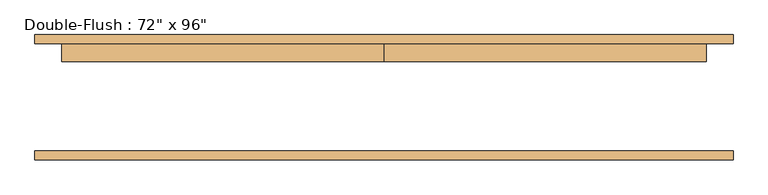
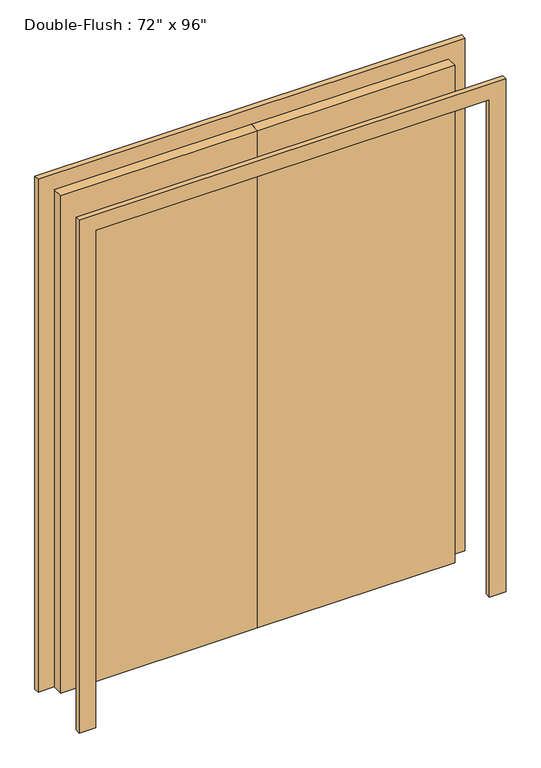
"""IFC4 building model written with IfcOpenShell, lengths in millimetres: door geometry."""

import ifcopenshell
import ifcopenshell.guid

model = None  # the IFC model being written
_history = None  # IfcOwnerHistory: only IFC2X3 demands one
_inside = {}  # id of a spatial element -> (the spatial element, [elements in it])
_under = {}  # id of a project, library or spatial element -> (it, [spatial elements below it])
_declared = {}  # id of a project -> (the project, [libraries it declares])
_typed = {}  # id of a type object -> (the type object, [elements of that type])
_made_of = {}  # id of a material, layer set ... -> (it, [elements and type objects made of it])


def new_model(schema):
    """Start an empty IFC model of exactly this schema.

    Asked for "IFC4X3", IfcOpenShell would pick the latest addendum, in which some entities
    have other attributes; the version numbers below select the first issue.
    IFC2X3 requires an IfcOwnerHistory on every rooted entity: one is made here for all.
    """
    global model, _history
    if schema == "IFC4X3":
        model = ifcopenshell.file(schema_version=(4, 3, 0, 0))
    else:
        model = ifcopenshell.file(schema=schema)
    _inside.clear()
    _under.clear()
    _declared.clear()
    _typed.clear()
    _made_of.clear()
    _history = None
    if model.schema == "IFC2X3":
        org = make("IfcOrganization", Name="unknown")
        user = make(
            "IfcPersonAndOrganization",
            ThePerson=make("IfcPerson", FamilyName="unknown"),
            TheOrganization=org,
        )
        app = make(
            "IfcApplication",
            ApplicationDeveloper=org,
            Version="unknown",
            ApplicationFullName="unknown",
            ApplicationIdentifier="unknown",
        )
        _history = make(
            "IfcOwnerHistory",
            OwningUser=user,
            OwningApplication=app,
            ChangeAction="ADDED",
            CreationDate=0,
        )
    return model


def make(cls, **values):
    """One entity of the class cls with the attributes given. An attribute that is None is left unset."""
    return model.create_entity(
        cls, **{name: value for name, value in values.items() if value is not None}
    )


def rooted(cls, **values):
    """An entity with a GlobalId (a new one), such as an element, a storey or a relation."""
    return make(cls, GlobalId=ifcopenshell.guid.new(), OwnerHistory=_history, **values)


def si_unit(unit_type, name, prefix=None):
    """IfcSIUnit, for example si_unit("LENGTHUNIT", "METRE", prefix="MILLI")."""
    return make("IfcSIUnit", UnitType=unit_type, Prefix=prefix, Name=name)


def assignment(units):
    """IfcUnitAssignment: the units of a project."""
    return None if units is None else make("IfcUnitAssignment", Units=units)


def point(xyz):
    """IfcCartesianPoint."""
    return None if xyz is None else make("IfcCartesianPoint", Coordinates=xyz)


def direction(xyz):
    """IfcDirection."""
    return None if xyz is None else make("IfcDirection", DirectionRatios=xyz)


def frame(location, z_axis=None, x_axis=None):
    """IfcAxis2Placement3D, a coordinate frame: its origin and axes. An axis left out is left unset."""
    return make(
        "IfcAxis2Placement3D",
        Location=point(location),
        Axis=direction(z_axis),
        RefDirection=direction(x_axis),
    )


def origin():
    """The frame at (0, 0, 0) with its axes left unset."""
    return frame((0.0, 0.0, 0.0))


def origin_with_axes():
    """The frame at (0, 0, 0) with the z axis (0, 0, 1) and the x axis (1, 0, 0) written out."""
    return frame((0.0, 0.0, 0.0), z_axis=(0.0, 0.0, 1.0), x_axis=(1.0, 0.0, 0.0))


def place(relative_to, where):
    """IfcLocalPlacement: puts the frame where relative to a parent placement (None: the world)."""
    return make(
        "IfcLocalPlacement", PlacementRelTo=relative_to, RelativePlacement=where
    )


def context(
    kind, dimensions, precision=None, world=None, true_north=None, identifier=None
):
    """IfcGeometricRepresentationContext, for example the 3D "Model" context."""
    return make(
        "IfcGeometricRepresentationContext",
        ContextIdentifier=identifier,
        ContextType=kind,
        CoordinateSpaceDimension=dimensions,
        Precision=precision,
        WorldCoordinateSystem=world,
        TrueNorth=true_north,
    )


def project(units=None, contexts=None):
    """IfcProject with its units and contexts."""
    return rooted(
        "IfcProject",
        Name="project",
        RepresentationContexts=contexts,
        UnitsInContext=assignment(units),
    )


def spatial(cls, under=None, at=None, **own):
    """A site, building, storey or space (cls), placed at a placement, below another one or the project."""
    s = rooted(cls, ObjectPlacement=at, **own)
    if under is not None:
        _under.setdefault(under.id(), (under, []))[1].append(s)
    return s


def polyline(points):
    """IfcPolyline through the points."""
    return make("IfcPolyline", Points=[point(p) for p in points])


def outline(outer, holes=None, kind="AREA"):
    """IfcArbitraryClosedProfileDef: a profile drawn as a closed curve; with holes, ...WithVoids."""
    if holes is None:
        return make("IfcArbitraryClosedProfileDef", ProfileType=kind, OuterCurve=outer)
    return make(
        "IfcArbitraryProfileDefWithVoids",
        ProfileType=kind,
        OuterCurve=outer,
        InnerCurves=holes,
    )


def extrude(swept, where, along, depth):
    """IfcExtrudedAreaSolid: the profile swept, set in the frame where, extruded along a direction by depth."""
    return make(
        "IfcExtrudedAreaSolid",
        SweptArea=swept,
        Position=where,
        ExtrudedDirection=direction(along),
        Depth=depth,
    )


def shape(context_of_items, identifier, shape_type, items):
    """IfcShapeRepresentation: the items that make up one representation, for example the "Body"."""
    return make(
        "IfcShapeRepresentation",
        ContextOfItems=context_of_items,
        RepresentationIdentifier=identifier,
        RepresentationType=shape_type,
        Items=items,
    )


def source(mapping_origin, context_of_items, identifier, shape_type, items):
    """IfcRepresentationMap: a shape defined once, which mapped items show again and again."""
    return make(
        "IfcRepresentationMap",
        MappingOrigin=mapping_origin,
        MappedRepresentation=shape(context_of_items, identifier, shape_type, items),
    )


def transform(
    local_origin,
    x_axis=None,
    y_axis=None,
    z_axis=None,
    scale=None,
    scale2=None,
    scale3=None,
    uniform=True,
):
    """IfcCartesianTransformationOperator3D, or its non-uniform kind. x_axis, y_axis, z_axis: its Axis1, 2, 3."""
    if uniform:
        return make(
            "IfcCartesianTransformationOperator3D",
            Axis1=direction(x_axis),
            Axis2=direction(y_axis),
            LocalOrigin=point(local_origin),
            Scale=scale,
            Axis3=direction(z_axis),
        )
    return make(
        "IfcCartesianTransformationOperator3DnonUniform",
        Axis1=direction(x_axis),
        Axis2=direction(y_axis),
        LocalOrigin=point(local_origin),
        Scale=scale,
        Axis3=direction(z_axis),
        Scale2=scale2,
        Scale3=scale3,
    )


def mapped(mapping_source, mapping_target):
    """IfcMappedItem: shows the shape of a source again, moved by a transform."""
    return make(
        "IfcMappedItem", MappingSource=mapping_source, MappingTarget=mapping_target
    )


def made_of(thing, what):
    """Note that an element or type object is made of a material, layer set ...; save() writes the relation."""
    if what is not None:
        _made_of.setdefault(what.id(), (what, []))[1].append(thing)
    return thing


def element(
    cls,
    number,
    at=None,
    inside=None,
    cuts=None,
    type_object=None,
    material=None,
    context=None,
    identifier="Body",
    shape_type=None,
    held_by="IfcProductDefinitionShape",
    body=None,
    shapes=None,
    **own,
):
    """One element of the class cls, such as IfcWall. Its Tag is "e" and its number.

    at: its placement. inside: the storey or other place that contains it. cuts: it is an
    opening in that element (IfcRelVoidsElement). A single representation is given by context,
    identifier, shape_type and body (its items); several are given by shapes. held_by: the class
    of the entity that holds the representations. save() writes the other relations.
    """
    e = rooted(cls, Tag="e%d" % number, ObjectPlacement=at, **own)
    if body is not None:
        shapes = [shape(context, identifier, shape_type, body)]
    if shapes is not None:
        e.Representation = make(held_by, Representations=shapes)
    if inside is not None:
        _inside.setdefault(inside.id(), (inside, []))[1].append(e)
    if cuts is not None:
        rooted(
            "IfcRelVoidsElement", RelatingBuildingElement=cuts, RelatedOpeningElement=e
        )
    if type_object is not None:
        _typed.setdefault(type_object.id(), (type_object, []))[1].append(e)
    return made_of(e, material)


def aggregate(whole, parts):
    """IfcRelAggregates: a whole, such as a stair, and the parts it consists of."""
    return rooted("IfcRelAggregates", RelatingObject=whole, RelatedObjects=parts)


def save(model, path):
    """Write the relations noted so far, then the file.

    IfcRelAggregates (storeys below a building ...), IfcRelContainedInSpatialStructure (elements
    in a storey), IfcRelDefinesByType, IfcRelAssociatesMaterial and IfcRelDeclares: one each for
    every whole, place, type object, material and project.
    """
    for whole, parts in _under.values():
        aggregate(whole, parts)
    for where, things in _inside.values():
        rooted(
            "IfcRelContainedInSpatialStructure",
            RelatedElements=things,
            RelatingStructure=where,
        )
    for kind, things in _typed.values():
        rooted("IfcRelDefinesByType", RelatedObjects=things, RelatingType=kind)
    for what, things in _made_of.values():
        rooted("IfcRelAssociatesMaterial", RelatedObjects=things, RelatingMaterial=what)
    for by, libraries in _declared.values():
        rooted("IfcRelDeclares", RelatingContext=by, RelatedDefinitions=libraries)
    model.write(path)


def door_6d7ee948(model_context):
    return source(origin(), model_context, "Body", "SweptSolid", [
        extrude(outline(polyline([(0.0, 152.4), (914.4, 152.4), (914.4, 101.6), (0.0, 101.6), (0.0, 152.4)])), origin_with_axes(), (0.0, 0.0, 1.0), 2438.4),
        extrude(outline(polyline([(-914.4, 152.4), (0.0, 152.4), (0.0, 101.6), (-914.4, 101.6), (-914.4, 152.4)])), origin_with_axes(), (0.0, 0.0, 1.0), 2438.4),
        extrude(outline(polyline([(2438.4, -914.4), (2438.4, 914.4), (0.0, 914.4), (0.0, 990.6), (2514.6, 990.6), (2514.6, -990.6), (0.0, -990.6), (0.0, -914.4), (2438.4, -914.4)])), frame((0.0, -177.8, 0.0), z_axis=(0.0, 1.0, 0.0), x_axis=(0.0, 0.0, 1.0)), (0.0, 0.0, 1.0), 25.4),
        extrude(outline(polyline([(2438.4, -914.4), (2438.4, 914.4), (0.0, 914.4), (0.0, 990.6), (2514.6, 990.6), (2514.6, -990.6), (0.0, -990.6), (0.0, -914.4), (2438.4, -914.4)])), frame((0.0, 152.4, 0.0), z_axis=(0.0, 1.0, 0.0), x_axis=(0.0, 0.0, 1.0)), (0.0, 0.0, 1.0), 25.4),
    ])


if __name__ == "__main__":
    model = new_model("IFC4")
    model_context = context("Model", 3, world=origin())
    ifc_project = project(units=[si_unit("LENGTHUNIT", "METRE", prefix="MILLI")], contexts=[model_context])
    site = spatial("IfcSite", under=ifc_project)
    building = spatial("IfcBuilding", under=site)
    placement = place(None, origin())
    door_shape = door_6d7ee948(model_context)
    element("IfcDoor", 1, ObjectType="Double-Flush : 72\" x 96\"", at=placement, inside=building, context=model_context, shape_type="MappedRepresentation", body=[
        mapped(door_shape, transform((0.0, 0.0, 0.0), x_axis=(1.0, 0.0, 0.0), y_axis=(0.0, 1.0, 0.0), z_axis=(0.0, 0.0, 1.0))),
    ])
    save(model, "model.ifc")

# Revit data of these elements
# Type "Double-Flush : 72\" x 96\""
#   Type Mark = "38"
#   Assembly Code = "C1020"
#   Thickness = 50.8 mm
#   Height = 2438.4 mm
#   Trim Projection Ext = 25.4 mm
#   Trim Projection Int = 25.4 mm
#   Trim Width = 76.2 mm
#   Width = 1828.8 mm
#   Door Material = Door - Panel
#   Frame Material = Door - Frame
#   Function = (empty or 0)
#   Wall Closure = (empty or 0)
# Element 1 (IfcDoor, "Double-Flush : 72\" x 96\"")
#   Materials on its faces: "Door - Frame", "Door - Panel"
# Materials
#   "Door - Panel": class "Wood", colour RGB 210 159 95, transparency 0
#   "Door - Frame": class "Miscellaneous", colour RGB 118 70 51, transparency 0
